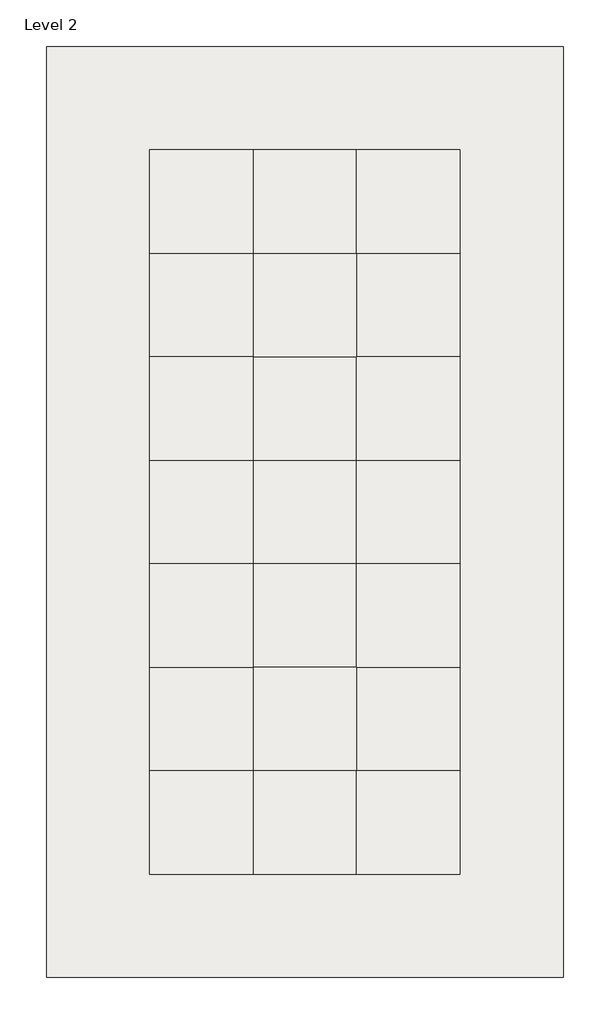
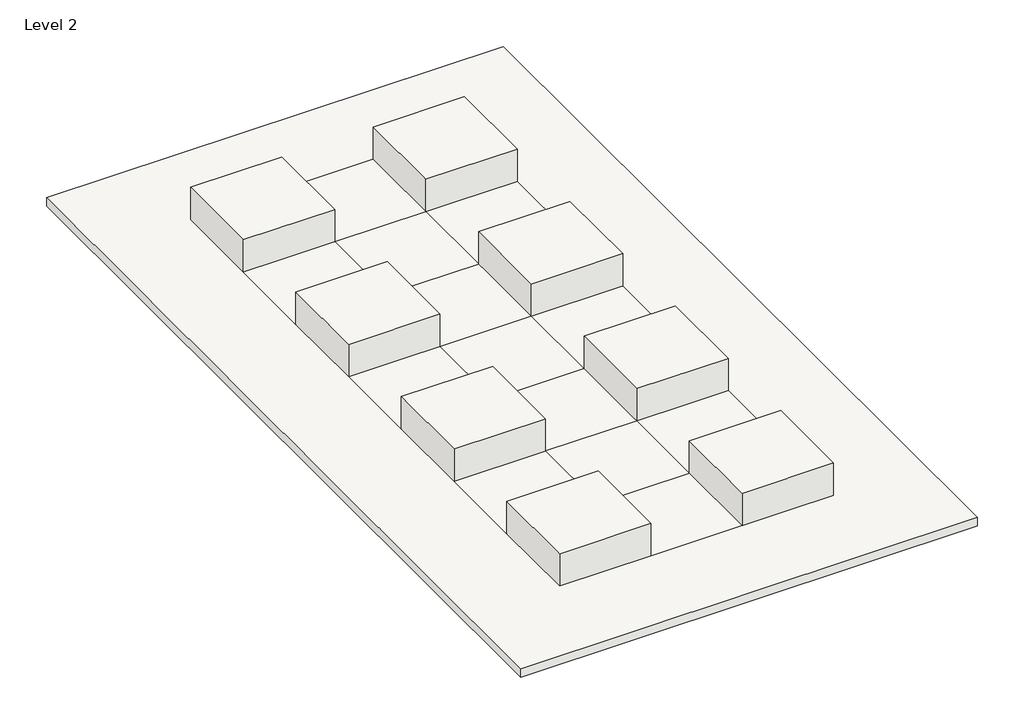
# One storey: 9 roofs.
"""IFC4 building model written with IfcOpenShell, lengths in millimetres."""

from ifc_helpers import new_model, si_unit, origin, place, context, project, spatial, faceted_brep, element, save

model = new_model("IFC4")

# Units and contexts
model_context = context("Model", 3, world=origin())
ifc_project = project(units=[si_unit("LENGTHUNIT", "METRE", prefix="MILLI")], contexts=[model_context])

# Site, building, storey
site = spatial("IfcSite", under=ifc_project)
building = spatial("IfcBuilding", under=site)
storey = spatial("IfcBuildingStorey", under=building, Name="Level 2", Elevation=8000.0)

# Roofs
placement = place(None, origin())
element("IfcRoof", 1, ObjectType="Bauder_RoofCoveringSystem_IntensiveGreenRoofSystem", at=placement, inside=storey, context=model_context, shape_type="Brep", body=[
    faceted_brep([(-674.7340554, 1676.2074539, 8000.0), (1325.2659446, 1676.2074539, 8000.0), (1325.2659446, -323.7925461, 8000.0), (-674.7340554, -323.7925461, 8000.0), (1325.2659446, 1676.2074539, 8949.8), (-674.7340554, 1676.2074539, 8949.8), (-674.7340554, -323.7925461, 8949.8), (1325.2659446, -323.7925461, 8949.8), (1325.2659446, 1676.2074539, 8200.0), (-674.7340554, 1676.2074539, 8200.0), (-674.7340554, -323.7925461, 8200.0), (1325.2659446, -323.7925461, 8200.0)], [[[0, 1, 2, 3]], [[4, 5, 6, 7]], [[5, 4, 8, 1, 0, 9]], [[6, 5, 9, 0, 3, 10]], [[7, 6, 10, 3, 2, 11]], [[4, 7, 11, 2, 1, 8]]]),
])
element("IfcRoof", 2, ObjectType="Bauder_RoofCoveringSystem_IntensiveGreenRoofSystem", at=placement, inside=storey, context=model_context, shape_type="Brep", body=[
    faceted_brep([(3325.2659446, 1676.2074539, 8000.0), (5325.2659446, 1676.2074539, 8000.0), (5325.2659446, -323.7925461, 8000.0), (3325.2659446, -323.7925461, 8000.0), (5325.2659446, 1676.2074539, 8949.8), (3325.2659446, 1676.2074539, 8949.8), (3325.2659446, -323.7925461, 8949.8), (5325.2659446, -323.7925461, 8949.8), (5325.2659446, 1676.2074539, 8200.0), (3325.2659446, 1676.2074539, 8200.0), (3325.2659446, -323.7925461, 8200.0), (5325.2659446, -323.7925461, 8200.0)], [[[0, 1, 2, 3]], [[4, 5, 6, 7]], [[5, 4, 8, 1, 0, 9]], [[6, 5, 9, 0, 3, 10]], [[7, 6, 10, 3, 2, 11]], [[4, 7, 11, 2, 1, 8]]]),
])
element("IfcRoof", 3, ObjectType="Bauder_RoofCoveringSystem_IntensiveGreenRoofSystem", at=placement, inside=storey, context=model_context, shape_type="Brep", body=[
    faceted_brep([(3325.2659446, -2323.7925461, 8000.0), (5325.2659446, -2323.7925461, 8000.0), (5325.2659446, -4323.7925461, 8000.0), (3325.2659446, -4323.7925461, 8000.0), (5325.2659446, -2323.7925461, 8949.8), (3325.2659446, -2323.7925461, 8949.8), (3325.2659446, -4323.7925461, 8949.8), (5325.2659446, -4323.7925461, 8949.8), (5325.2659446, -2323.7925461, 8200.0), (3325.2659446, -2323.7925461, 8200.0), (3325.2659446, -4323.7925461, 8200.0), (5325.2659446, -4323.7925461, 8200.0)], [[[0, 1, 2, 3]], [[4, 5, 6, 7]], [[5, 4, 8, 1, 0, 9]], [[6, 5, 9, 0, 3, 10]], [[7, 6, 10, 3, 2, 11]], [[4, 7, 11, 2, 1, 8]]]),
])
element("IfcRoof", 4, ObjectType="Bauder_RoofCoveringSystem_IntensiveGreenRoofSystem", at=placement, inside=storey, context=model_context, shape_type="Brep", body=[
    faceted_brep([(3325.2659446, -6323.7925461, 8000.0), (5325.2659446, -6323.7925461, 8000.0), (5325.2659446, -8323.7925461, 8000.0), (3325.2659446, -8323.7925461, 8000.0), (5325.2659446, -6323.7925461, 8949.8), (3325.2659446, -6323.7925461, 8949.8), (3325.2659446, -8323.7925461, 8949.8), (5325.2659446, -8323.7925461, 8949.8), (5325.2659446, -6323.7925461, 8200.0), (3325.2659446, -6323.7925461, 8200.0), (3325.2659446, -8323.7925461, 8200.0), (5325.2659446, -8323.7925461, 8200.0)], [[[0, 1, 2, 3]], [[4, 5, 6, 7]], [[5, 4, 8, 1, 0, 9]], [[6, 5, 9, 0, 3, 10]], [[7, 6, 10, 3, 2, 11]], [[4, 7, 11, 2, 1, 8]]]),
])
element("IfcRoof", 5, ObjectType="Bauder_RoofCoveringSystem_IntensiveGreenRoofSystem", at=placement, inside=storey, context=model_context, shape_type="Brep", body=[
    faceted_brep([(3325.2659446, -10323.7925461, 8000.0), (5325.2659446, -10323.7925461, 8000.0), (5325.2659446, -12323.7925461, 8000.0), (3325.2659446, -12323.7925461, 8000.0), (5325.2659446, -10323.7925461, 8949.8), (3325.2659446, -10323.7925461, 8949.8), (3325.2659446, -12323.7925461, 8949.8), (5325.2659446, -12323.7925461, 8949.8), (5325.2659446, -10323.7925461, 8200.0), (3325.2659446, -10323.7925461, 8200.0), (3325.2659446, -12323.7925461, 8200.0), (5325.2659446, -12323.7925461, 8200.0)], [[[0, 1, 2, 3]], [[4, 5, 6, 7]], [[5, 4, 8, 1, 0, 9]], [[6, 5, 9, 0, 3, 10]], [[7, 6, 10, 3, 2, 11]], [[4, 7, 11, 2, 1, 8]]]),
])
element("IfcRoof", 6, ObjectType="Bauder_RoofCoveringSystem_IntensiveGreenRoofSystem", at=placement, inside=storey, context=model_context, shape_type="Brep", body=[
    faceted_brep([(-674.7340554, -10323.7925461, 8000.0), (1325.2659446, -10323.7925461, 8000.0), (1325.2659446, -12323.7925461, 8000.0), (-674.7340554, -12323.7925461, 8000.0), (1325.2659446, -10323.7925461, 8949.8), (-674.7340554, -10323.7925461, 8949.8), (-674.7340554, -12323.7925461, 8949.8), (1325.2659446, -12323.7925461, 8949.8), (1325.2659446, -10323.7925461, 8200.0), (-674.7340554, -10323.7925461, 8200.0), (-674.7340554, -12323.7925461, 8200.0), (1325.2659446, -12323.7925461, 8200.0)], [[[0, 1, 2, 3]], [[4, 5, 6, 7]], [[5, 4, 8, 1, 0, 9]], [[6, 5, 9, 0, 3, 10]], [[7, 6, 10, 3, 2, 11]], [[4, 7, 11, 2, 1, 8]]]),
])
element("IfcRoof", 7, ObjectType="Bauder_RoofCoveringSystem_IntensiveGreenRoofSystem", at=placement, inside=storey, context=model_context, shape_type="Brep", body=[
    faceted_brep([(-674.7340554, -6323.7925461, 8000.0), (1325.2659446, -6323.7925461, 8000.0), (1325.2659446, -8323.7925461, 8000.0), (-674.7340554, -8323.7925461, 8000.0), (1325.2659446, -6323.7925461, 8949.8), (-674.7340554, -6323.7925461, 8949.8), (-674.7340554, -8323.7925461, 8949.8), (1325.2659446, -8323.7925461, 8949.8), (1325.2659446, -6323.7925461, 8200.0), (-674.7340554, -6323.7925461, 8200.0), (-674.7340554, -8323.7925461, 8200.0), (1325.2659446, -8323.7925461, 8200.0)], [[[0, 1, 2, 3]], [[4, 5, 6, 7]], [[5, 4, 8, 1, 0, 9]], [[6, 5, 9, 0, 3, 10]], [[7, 6, 10, 3, 2, 11]], [[4, 7, 11, 2, 1, 8]]]),
])
element("IfcRoof", 8, ObjectType="Bauder_RoofCoveringSystem_IntensiveGreenRoofSystem", at=placement, inside=storey, context=model_context, shape_type="Brep", body=[
    faceted_brep([(-674.7340554, -2323.7925461, 8000.0), (1325.2659446, -2323.7925461, 8000.0), (1325.2659446, -4323.7925461, 8000.0), (-674.7340554, -4323.7925461, 8000.0), (1325.2659446, -2323.7925461, 8949.8), (-674.7340554, -2323.7925461, 8949.8), (-674.7340554, -4323.7925461, 8949.8), (1325.2659446, -4323.7925461, 8949.8), (1325.2659446, -2323.7925461, 8200.0), (-674.7340554, -2323.7925461, 8200.0), (-674.7340554, -4323.7925461, 8200.0), (1325.2659446, -4323.7925461, 8200.0)], [[[0, 1, 2, 3]], [[4, 5, 6, 7]], [[5, 4, 8, 1, 0, 9]], [[6, 5, 9, 0, 3, 10]], [[7, 6, 10, 3, 2, 11]], [[4, 7, 11, 2, 1, 8]]]),
])
element("IfcRoof", 9, ObjectType="Roof_Concrete-200mm", at=placement, inside=storey, context=model_context, shape_type="Brep", body=[
    faceted_brep([(-2674.7340554, -14323.7925461, 8200.0), (-2674.7340554, -14323.7925461, 8000.0), (7325.2659446, -14323.7925461, 8000.0), (7325.2659446, -14323.7925461, 8200.0), (-2674.7340554, 3676.2074539, 8200.0), (-2674.7340554, 3676.2074539, 8000.0), (7325.2659446, 3676.2074539, 8200.0), (7325.2659446, 3676.2074539, 8000.0), (3325.2659446, 1676.2074539, 8200.0), (1325.2659446, 1676.2074539, 8200.0), (1325.2659446, -323.7925461, 8200.0), (3325.2659446, -323.7925461, 8200.0), (1325.2659446, 1676.2074539, 8000.0), (3325.2659446, 1676.2074539, 8000.0), (3325.2659446, -323.7925461, 8000.0), (1325.2659446, -323.7925461, 8000.0), (1325.2659446, -2323.7925461, 8200.0), (-674.7340554, -323.7925461, 8200.0), (-674.7340554, -2323.7925461, 8200.0), (3325.2659446, -2323.7925461, 8200.0), (5325.2659446, -2323.7925461, 8200.0), (5325.2659446, -323.7925461, 8200.0), (-674.7340554, -2323.7925461, 8000.0), (-674.7340554, -323.7925461, 8000.0), (1325.2659446, -2323.7925461, 8000.0), (3325.2659446, -2323.7925461, 8000.0), (5325.2659446, -323.7925461, 8000.0), (5325.2659446, -2323.7925461, 8000.0), (1325.2659446, -4323.7925461, 8200.0), (3325.2659446, -4323.7925461, 8200.0), (3325.2659446, -4323.7925461, 8000.0), (1325.2659446, -4323.7925461, 8000.0), (1325.2659446, -6323.7925461, 8200.0), (-674.7340554, -4323.7925461, 8200.0), (-674.7340554, -6323.7925461, 8200.0), (5325.2659446, -6323.7925461, 8200.0), (5325.2659446, -4323.7925461, 8200.0), (3325.2659446, -6323.7925461, 8200.0), (-674.7340554, -6323.7925461, 8000.0), (-674.7340554, -4323.7925461, 8000.0), (1325.2659446, -6323.7925461, 8000.0), (3325.2659446, -6323.7925461, 8000.0), (5325.2659446, -4323.7925461, 8000.0), (5325.2659446, -6323.7925461, 8000.0), (1325.2659446, -12323.7925461, 8200.0), (3325.2659446, -12323.7925461, 8200.0), (3325.2659446, -10323.7925461, 8200.0), (1325.2659446, -10323.7925461, 8200.0), (3325.2659446, -12323.7925461, 8000.0), (1325.2659446, -12323.7925461, 8000.0), (1325.2659446, -10323.7925461, 8000.0), (3325.2659446, -10323.7925461, 8000.0), (1325.2659446, -8323.7925461, 8200.0), (-674.7340554, -8323.7925461, 8200.0), (-674.7340554, -10323.7925461, 8200.0), (3325.2659446, -8323.7925461, 8200.0), (5325.2659446, -10323.7925461, 8200.0), (5325.2659446, -8323.7925461, 8200.0), (-674.7340554, -10323.7925461, 8000.0), (-674.7340554, -8323.7925461, 8000.0), (1325.2659446, -8323.7925461, 8000.0), (3325.2659446, -8323.7925461, 8000.0), (5325.2659446, -8323.7925461, 8000.0), (5325.2659446, -10323.7925461, 8000.0), (-674.7340554, 1676.2074539, 8000.0), (-674.7340554, 1676.2074539, 8200.0), (5325.2659446, 1676.2074539, 8200.0), (5325.2659446, 1676.2074539, 8000.0), (5325.2659446, -12323.7925461, 8000.0), (5325.2659446, -12323.7925461, 8200.0), (-674.7340554, -12323.7925461, 8000.0), (-674.7340554, -12323.7925461, 8200.0)], [[[0, 1, 2, 3]], [[1, 0, 4, 5]], [[6, 7, 5, 4]], [[3, 2, 7, 6]], [[8, 9, 10, 11]], [[12, 13, 14, 15]], [[16, 10, 17, 18]], [[11, 10, 16, 19]], [[20, 21, 11, 19]], [[22, 23, 15, 24]], [[15, 14, 25, 24]], [[25, 14, 26, 27]], [[19, 16, 28, 29]], [[24, 25, 30, 31]], [[32, 28, 33, 34]], [[35, 36, 29, 37]], [[38, 39, 31, 40]], [[41, 30, 42, 43]], [[44, 45, 46, 47]], [[48, 49, 50, 51]], [[47, 52, 53, 54]], [[47, 46, 55, 52]], [[56, 57, 55, 46]], [[58, 59, 60, 50]], [[51, 50, 60, 61]], [[51, 61, 62, 63]], [[52, 55, 37, 32]], [[29, 28, 32, 37]], [[61, 60, 40, 41]], [[31, 30, 41, 40]], [[9, 12, 15, 10]], [[10, 15, 23, 17]], [[17, 23, 64, 65]], [[12, 9, 65, 64]], [[66, 67, 26, 21]], [[21, 26, 14, 11]], [[11, 14, 13, 8]], [[67, 66, 8, 13]], [[20, 27, 42, 36]], [[36, 42, 30, 29]], [[29, 30, 25, 19]], [[27, 20, 19, 25]], [[16, 24, 31, 28]], [[28, 31, 39, 33]], [[33, 39, 22, 18]], [[24, 16, 18, 22]], [[32, 40, 60, 52]], [[52, 60, 59, 53]], [[53, 59, 38, 34]], [[40, 32, 34, 38]], [[35, 43, 62, 57]], [[57, 62, 61, 55]], [[55, 61, 41, 37]], [[43, 35, 37, 41]], [[56, 63, 68, 69]], [[69, 68, 48, 45]], [[45, 48, 51, 46]], [[63, 56, 46, 51]], [[47, 50, 49, 44]], [[44, 49, 70, 71]], [[71, 70, 58, 54]], [[50, 47, 54, 58]], [[4, 0, 3, 6], [9, 8, 66, 21, 20, 36, 35, 57, 56, 69, 45, 44, 71, 54, 53, 34, 33, 18, 17, 65]], [[7, 2, 1, 5], [13, 12, 64, 23, 22, 39, 38, 59, 58, 70, 49, 48, 68, 63, 62, 43, 42, 27, 26, 67]]]),
])

save(model, "model.ifc")

# Revit data of these elements
# Type "Bauder_RoofCoveringSystem_IntensiveGreenRoofSystem"
#   Keynote = "Q37"
#   Type IFC Predefined Type = "FLAT_ROOF"
#   Export Type to IFC As = "IfcRoofType"
#   Model = "Bauder Intensive Landscaping and Substrate - Intensive Green Roof System"
#   Manufacturer = "Bauder Ltd"
#   Type Comments = "Intensive Green Roof System"
#   URL = "http://www.bauder.co.uk/"
#   Description = "Bauder Intensive GreenRoof system incorporating Intensive Landscaping with Intensive Substrate, Filter Fleece, Mineral Drain, DSE60 Polyethylene Drainage and Protection Layer, FSM 1100 protection mat and PE Foil Polyethylene Separation-Slip Layer"
#   Assembly Code = "B3010"
#   NBSDescription = "Intensive green roof system"
#   NBSReference = "45-40-47/110"
#   BIMObjectName = "Bauder_RoofCoveringSystem_IntensiveGreenRoofSystem"
#   AccessibilityPerformance = "n/a"
#   CodePerformance = "n/a"
#   Color = "n/a"
#   Constituents = "n/a"
#   DurationUnit = "Year"
#   ExpectedLife = "n/a"
#   Features = "This BIM Object must be supported by a project specific specification from Bauder, incorporating system build-up, detail design and performance calculations if a full Bauder system guarantee is required. Please contact your local Bauder Representative or technical@bauder.co.uk"
#   Finish = "n/a"
#   Grade = "n/a"
#   Material = "n/a"
#   ModelReference = "Bauder Intensive Landscaping and Substrate - Intensive Green Roof System"
#   Name = "RoofCoveringSystem_Bauder_IntensiveGreenRoofSystem"
#   ReplacementCost = "n/a"
#   Shape = "n/a"
#   Size = "n/a"
#   SustainabilityPerformance = "Bauder Germany ISO14001: Certificate No.: 70499/03-15 e, Bauder UK ISO14001:Certificate No. 19ACM6595R, EN1271, BREEAM Credits Available"
#   WarrantyDescription = "Guarantee options could include ‘Product’, ‘Product and Workmanship’ and ‘Product, Workmanship and Design’ Guarantees. All guarantees available for this system are subject to the works being carried out in accordance with the Bauder specification and being installed by a Bauder Approved installer. For full details and further information regarding guarantees and alternative systems please contact your local Bauder Representative or technical@bauder.co.uk"
#   WarrantyDurationLabor = "n/a"
#   WarrantyDurationParts = "n/a\r\nn/a"
#   WarrantyDurationUnit = "Year"
#   WarrantyGuarantorLabor = "n/a"
#   WarrantyGuarantorParts = "technical@bauder.co.uk"
#   Certification = "n/a"
#   EdgeRestraints = "Perforated edge trim where required, refer to Bauder Project Specific Specification"
#   MoistureControlDrainageAncillaries = "n/a"
#   MoistureControlDrainageLayer = "Bauder DSE60 60 mm Polyethylene Drainage and Protection Layer with Bauder Mineral Drain Single size stone aggregate infill"
#   MoistureControlFilterMembrane = "Bauder Filter Fleece 1 mm Polypropylene Filter Fleece"
#   MoistureControlMoistureRetentionMat = "n/a"
#   PlantingSystemsAntierosionMat = "Jute Net where exposed, refer to Bauder Project Specific Specification"
#   PlantingSystemsPlantingMedium = "Bauder Intensive Substrate Recycled crushed brick, expanded clay shale and composted pine bark"
#   PlantingSystemsVegetation = "Bauder Intensive Landscaping"
#   PlantingSystemsVegetationBarrier = "20-40 mm Rounded-Washed Stones, refer to Bauder Project Specific Specification"
#   ProjectSpecificationAndDesign = "This BIM Object must be supported by a project specific specification from Bauder, incorporating system build-up, detail design and performance calculations if a full Bauder system warranty is required. Please contact your local Bauder Representative or technical@bauder.co.uk"
#   ProtectionProtectionLayer = "BauderGREEN FSM 1100 Protection Mat"
#   ProtectionRootBarrier = "As per project specific Bauder Specification"
#   ProtectionSeparationLayer = "2 layers of Bauder PE Foil 0.2 mm Polyethylene Separation-Slip Layer"
#   SystemManufacturer = "Bauder Ltd"
#   WarrantyConsiderations = "All guarantees available for this system are subject to the works being carried out in accordance with the Bauder specification and being installed by a Bauder Approved installer. For full details and further information regarding guarantees and alternative systems please contact your local Bauder Representative or technical@bauder.co.uk"
#   Update = "1900-12-31T23:59:59"
#   Documentation = "https://www.bauder.co.uk/technical-centre/technical-literature/system-brochures"
#   DocumentReference = "http://www.bauder.co.uk/"
#   IfcExportAs = "IfcRoofType"
#   IfcExportType = "FLAT_ROOF"
#   MethodOfMesurement = "n/a"
#   Process = "Replacement at service life intervals"
#   FireRating = "n/a"
#   _Author = "AM"
#   _AuthorizedBy = "bimstore"
#   _CreatedBy = "technical@bauder.co.uk"
#   _DistributedBy = "www.bimstore.co"
#   AssetType = "Fixed"
#   ClassificationName = "Uniclass2015"
#   ClassificationValue = "Ss_45_40_47_40"
#   CreatedBy = "technical@bauder.co.uk"
#   CreatedOn = "2023-02-10 T00:00:00"
#   DocumentationCertificates = "n/a"
#   DocumentationInstallationGuide = "https://www.bauder.co.uk/technical-centre"
#   DocumentationLiterature = "https://www.bauder.co.uk/technical-centre"
#   DocumentationMaintenance = "https://www.bauder.co.uk/technical-centre/maintenance-advice"
#   DocumentationTechnical = "https://www.bauder.co.uk/green-roofs/intensive-green-roofs"
#   ManufacturerName = "Bauder Ltd"
#   ModelNumber = "0910_INT-InS-FF-D6-F11-PE"
#   ProductionYear = "2023"
#   ReferencedStandard = "n/a"
#   SpareParts = "n/a"
#   TypeName = "Intensive Green Roof System"
#   NBSNote = "n/a"
#   NBSObjectName = "Bauder - Intensive green roof system"
#   NBSOfficeMasterTag = "n/a"
#   Ballast = "n/a"
#   CarrierMembraneFixing = "n/a"
#   CarrierMembraneType = "n/a"
#   FillToPerimeterUpstands = "n/a"
#   FilterLayer = "n/a"
#   InsulationFixing = "n/a"
#   InsulationType = "n/a"
#   LiquidAppliedWaterproofCoatingReinforcement = "n/a"
#   LiquidAppliedWaterproofCoatingSurfaceTreatment = "n/a"
#   LiquidAppliedWaterproofCoatingType = "n/a"
#   PreparationExistingSubstrates = "n/a"
#   PreparationHorizontalWork = "n/a"
#   PreparationSkirtingsAndVerticalWork = "n/a"
#   ProtectionLayer = "n/a"
#   SystemAccessories = "n/a"
#   WaterproofCoveringFirstLayerAttachment = "n/a"
#   WaterproofCoveringFirstLayerType = "n/a"
#   WaterproofCoveringIntermediateLayerAttachment = "n/a"
#   WaterproofCoveringIntermediateLayerType = "n/a"
#   WaterproofCoveringTopLayerAttachment = "n/a"
#   InsulationAttachment = "n/a"
#   IsolatingLayer = "n/a"
#   CarrierMembraneAttachment = "n/a"
#   LiquidAppliedWaterproofCoatingWearingCourse = "n/a"
#   VapourControlLayer = "n/a"
#   VapourControlLayerAttachment_Bauder = "n/a"
#   WaterproofCoveringJoints = "n/a"
#   WaterproofCoveringType = "n/a"
#   SeparatingLayer = "n/a"
#   WaterproofCoveringAccessories = "Yes"
#   WaterproofCoveringAttachment = "n/a"
#   UpperProtectionLayer = "n/a"
#   LowerProtectionLayer = "n/a"
#   WaterproofCoveringTopLayerType = "n/a"
#   DetailWorkAncillaryItems = "Detail as per project specific Bauder Specification"
#   DetailWorkCoverStrips = "Detail as per project specific Bauder Specification"
#   DetailWorkFlashings = "Detail as per project specific Bauder Specification"
#   DetailWorkSkirtingsAndUpstands = "Detail as per project specific Bauder Specification"
#   DetailWorkWeltedDrips = "Detail as per project specific Bauder Specification"
#   OverlayFixing = "n/a"
#   OverlayType = "n/a"
#   SurfaceProtection = "n/a"
#   VapourControlLayerAttachment = "n/a"
#   VapourControlLayerType = "n/a"
#   Cost = 0
#   NominalHeight = 0 mm
#   NominalLength = 0 mm
#   TotalArea = 0 m²
#   NominalDepth = 0 mm
#   IsExternal = yes
#   _BimSpecGuid = 0
#   _BSBibleVersion = 16
#   _CurrentRevision = 4
#   Layers, outside or top first: 300 mm "Bauder_Landscaping_Intensive" (function 5); 400 mm "Bauder_IntensiveSubstrate_BauderGREEN-SUB-IM-UK" (function 2); 1 mm "Bauder_FilterFleece_BauderGREEN-FV-125-100" (function 2); 40 mm "Bauder_DrainageBoard_BauderGREEN-DSE-40" (function 3); 8 mm "Bauder_ProtectionMat_BauderGREEN-FSM1100" (function 3); 200 mm "Concrete" (function 1); 0.8 mm "Bauder_SeparationAndSlipLayer_BauderGREEN-PE-02" (function 3)
# Type "Roof_Concrete-200mm"
#   Layers, outside or top first: 200 mm "Concrete" (function 1)
# Elements 1, 2, 3, 4, 5, 6, 7, 8 (IfcRoof, "Bauder_RoofCoveringSystem_IntensiveGreenRoofSystem")
#   built-in parameter 1001705 = 29.3629 (stored number, unit not read)
#   built-in parameter 1001710 = 33615
#   Phase Created = New Construction
#   Materials on its faces: "Bauder_SeparationAndSlipLayer_BauderGREEN-PE-02", "Bauder_Landscaping_Intensive"
# Element 9 (IfcRoof, "Roof_Concrete-200mm")
#   built-in parameter 1001710 = 33615
#   Phase Created = New Construction
#   Materials on its faces: "Concrete"
# Materials
#   "Bauder_Landscaping_Intensive": class "Unassigned", colour RGB 62 68 37, transparency 0, Mtrl_Author = "AM", Mtrl_AuthorizedBy = "bimstore", Mtrl_DistributedBy = "www.bimstore.co", Mtrl_AccessibilityPerformance = "n/a", Mtrl_AssetIdentifier = "Please record on commissioning", Mtrl_AssetType = "Fixed", Mtrl_BarCode = "Please record on commissioning", Mtrl_ClassificationName = "Uniclass2015", Mtrl_ClassificationValue = "n/a", Mtrl_CodePerformance = "n/a", Mtrl_Color = "n/a", Mtrl_Constituents = "n/a", Mtrl_CreatedBy = "technical@bauder.co.uk", Mtrl_CreatedOn = "2023-02-10 T00:00:00", Mtrl_DocumentationCertificates = "https://www.bimstore.co/products/intensive-green-roof-system/document/product-certificates", Mtrl_DocumentationInstallationGuide = "https://www.bimstore.co/products/intensive-green-roof-system/document/installation-guide", Mtrl_DocumentationLiterature = "https://www.bimstore.co/products/intensive-green-roof-system/document/product-literature", Mtrl_DocumentationMaintenance = "https://www.bimstore.co/products/intensive-green-roof-system/document/maintenance-information", Mtrl_DocumentationTechnical = "https://www.bimstore.co/products/intensive-green-roof-system/document/technical-data-sheet", Mtrl_DurationUnit = "Year", Mtrl_Features = "n/a", Mtrl_Finish = "n/a", Mtrl_Grade = "n/a", Mtrl_InstallationDate = "Please record on commissioning", Mtrl_ManufacturerName = "Bauder Ltd", Mtrl_Material = "n/a", Mtrl_ModelNumber = "Intensive", Mtrl_ModelReference = "Landscaping", Mtrl_ProductionYear = "2023", Mtrl_ReferencedStandard = "n/a", Mtrl_Shape = "n/a", Mtrl_Size = "n/a", Mtrl_SpareParts = "n/a", Mtrl_TypeName = "Intensive", Mtrl_WarrantyDescription = "n/a", Mtrl_WarrantyDurationUnit = "Year", Mtrl_WarrantyGuarantorLabor = "n/a", Mtrl_WarrantyGuarantorParts = "technical@bauder.co.uk", Mtrl_WarrantyStartDate = "Please record on commissioning", Mtrl_IfcExportAs = "IfcRoofType", Mtrl_IfcExportType = "FLAT_ROOF", Mtrl_BIMObjectName = "Bauder_Landscaping_Intensive", Mtrl_NBSDescription = "n/a", Mtrl_NBSNote = "n/a", Mtrl_NBSObjectName = "n/a", Mtrl_NBSOfficeMasterTag = "n/a", Mtrl_NBSReference = "Q37", Mtrl_Ballast = "n/a", Mtrl_CarrierMembraneAttachment = "n/a", Mtrl_CarrierMembraneFixing = "n/a", Mtrl_CarrierMembraneType = "n/a", Mtrl_Certification = "Comply with GRO Green Roof Code of Practice and FLL Standards", Mtrl_DetailWorkAncillaryItems = "Detail as per project specific Bauder Specification", Mtrl_DetailWorkCoverStrips = "Detail as per project specific Bauder Specification", Mtrl_DetailWorkFlashings = "Detail as per project specific Bauder Specification", Mtrl_DetailWorkSkirtingsAndUpstands = "Detail as per project specific Bauder Specification", Mtrl_DetailWorkWeltedDrips = "Detail as per project specific Bauder Specification", Mtrl_EdgeRestraints = "Detail as per project specific Bauder Specification", Mtrl_FillToPerimeterUpstands = "n/a", Mtrl_FilterLayer = "n/a", Mtrl_InsulationAttachment = "As per project specific Bauder Specification", Mtrl_InsulationFixing = "As per project specific Bauder Specification", Mtrl_InsulationType = "As per project specific Bauder Specification", Mtrl_IsolatingLayer = "n/a", Mtrl_LiquidAppliedWaterproofCoatingReinforcement = "n/a", Mtrl_LiquidAppliedWaterproofCoatingSurfaceTreatment = "As per project specific Bauder Specification", Mtrl_LiquidAppliedWaterproofCoatingType = "As per project specific Bauder Specification", Mtrl_LiquidAppliedWaterproofCoatingWearingCourse = "As per project specific Bauder Specification", Mtrl_LowerProtectionLayer = "n/a", Mtrl_MoistureControlDrainageAncillaries = "n/a", Mtrl_MoistureControlDrainageLayer = "n/a", Mtrl_MoistureControlFilterMembrane = "n/a", Mtrl_MoistureControlMoistureRetentionMat = "n/a", Mtrl_OverlayFixing = "n/a", Mtrl_OverlayType = "n/a", Mtrl_PlantingSystemsAntierosionMat = "n/a", Mtrl_PlantingSystemsPlantingMedium = "As per project specific Bauder Specification", Mtrl_PlantingSystemsVegetation = "As per project specific Bauder Specification", Mtrl_PlantingSystemsVegetationBarrier = "As per project specific Bauder Specification", Mtrl_PreparationExistingSubstrates = "n/a", Mtrl_PreparationHorizontalWork = "n/a", Mtrl_PreparationSkirtingsAndVerticalWork = "n/a", Mtrl_ProjectSpecificationAndDesign = "This BIM Object must be supported by a project specific specification from Bauder, incorporating system build-up, detail design and performance calculations if a full Bauder system warranty is required. Please contact your local Bauder Representative or technical@bauder.co.uk", Mtrl_ProtectionLayer = "n/a", Mtrl_ProtectionProtectionLayer = "n/a", Mtrl_ProtectionRootBarrier = "As per project specific Bauder Specification", Mtrl_ProtectionSeparationLayer = "n/a", Mtrl_SeparatingLayer = "n/a", Mtrl_SurfaceProtection = "n/a", Mtrl_SystemAccessories = "n/a", Mtrl_SystemManufacturer = "Bauder Ltd", Mtrl_Update = "1900-12-31 T23:59:59", Mtrl_UpperProtectionLayer = "n/a", Mtrl_VapourControlLayerAttachment = "As per project specific Bauder Specification", Mtrl_VapourControlLayerAttachment_Bauder = "As per project specific Bauder Specification", Mtrl_VapourControlLayerType = "As per project specific Bauder Specification", Mtrl_WarrantyConsiderations = "All guarantees available for this system are subject to the works being carried out in accordance with the Bauder specification and being installed by a Bauder Approved installer. For full details and further information regarding guarantees and alternative systems please contact your local Bauder Representative or technical@bauder.co.uk", Mtrl_WaterproofCoveringAccessories = "As per project specific Bauder Specification", Mtrl_WaterproofCoveringAttachment = "As per project specific Bauder Specification", Mtrl_WaterproofCoveringFirstLayerAttachment = "As per project specific Bauder Specification", Mtrl_WaterproofCoveringFirstLayerType = "As per project specific Bauder Specification", Mtrl_WaterproofCoveringIntermediateLayerAttachment = "As per project specific Bauder Specification", Mtrl_WaterproofCoveringIntermediateLayerType = "As per project specific Bauder Specification", Mtrl_WaterproofCoveringJoints = "As per project specific Bauder Specification", Mtrl_WaterproofCoveringTopLayerAttachment = "As per project specific Bauder Specification", Mtrl_WaterproofCoveringTopLayerType = "As per project specific Bauder Specification", Mtrl_WaterproofCoveringType = "As per project specific Bauder Specification", Cost = 0, Mtrl_ReplacementCost = 0, Mtrl_NominalDepth = 0 mm, Mtrl_NominalHeight = 0 mm, Mtrl_NominalLength = 0 mm, Mtrl_BimSpecGuid = 0, Mtrl_BSBibleVersion = 17, Mtrl_CurrentRevision = 2, Mtrl_ExpectedLife = 0, Mtrl_SerialNumber = 0, Mtrl_WarrantyDurationLabor = 0, Mtrl_WarrantyDurationParts = 0
#   "Bauder_IntensiveSubstrate_BauderGREEN-SUB-IM-UK": class "Unassigned", colour RGB 255 255 255, transparency 0, Mtrl_Author = "AM", Mtrl_AuthorizedBy = "bimstore", Mtrl_DistributedBy = "www.bimstore.co", Mtrl_AccessibilityPerformance = "n/a", Mtrl_AssetIdentifier = "Please record on commissioning", Mtrl_AssetType = "Fixed", Mtrl_BarCode = "Please record on commissioning", Mtrl_ClassificationName = "Uniclass2015", Mtrl_ClassificationValue = "n/a", Mtrl_CodePerformance = "n/a", Mtrl_Color = "n/a", Mtrl_Constituents = "n/a", Mtrl_CreatedBy = "technical@bauder.co.uk", Mtrl_CreatedOn = "2023-02-10 T00:00:00", Mtrl_DocumentationCertificates = "https://www.bimstore.co/products/intensive-green-roof-system/document/product-certificates", Mtrl_DocumentationInstallationGuide = "https://www.bimstore.co/products/intensive-green-roof-system/document/installation-guide", Mtrl_DocumentationLiterature = "https://www.bimstore.co/products/intensive-green-roof-system/document/product-literature", Mtrl_DocumentationMaintenance = "https://www.bimstore.co/products/intensive-green-roof-system/document/maintenance-information", Mtrl_DocumentationTechnical = "https://www.bimstore.co/products/intensive-green-roof-system/document/technical-data-sheet", Mtrl_DurationUnit = "Year", Mtrl_Features = "n/a", Mtrl_Finish = "n/a", Mtrl_Grade = "n/a", Mtrl_InstallationDate = "Please record on commissioning", Mtrl_ManufacturerName = "Bauder Ltd", Mtrl_Material = "Expanded Clay Aggregate", Mtrl_ModelNumber = "BauderGREEN-SUB-IM-UK", Mtrl_ModelReference = "Intensive Substrate", Mtrl_ProductionYear = "2023", Mtrl_ReferencedStandard = "n/a", Mtrl_Shape = "n/a", Mtrl_Size = "n/a", Mtrl_SpareParts = "n/a", Mtrl_TypeName = "BauderGREEN-SUB-IM-UK", Mtrl_WarrantyDescription = "As part of Bauder system guarantee, per specification", Mtrl_WarrantyDurationUnit = "Year", Mtrl_WarrantyGuarantorLabor = "n/a", Mtrl_WarrantyGuarantorParts = "technical@bauder.co.uk", Mtrl_WarrantyStartDate = "Please record on commissioning", Mtrl_IfcExportAs = "IfcRoofType", Mtrl_IfcExportType = "FLAT_ROOF", Mtrl_BIMObjectName = "Bauder_IntensiveSubstrate_BauderGREEN-SUB-IM-UK", Mtrl_NBSDescription = "n/a", Mtrl_NBSNote = "n/a", Mtrl_NBSObjectName = "n/a", Mtrl_NBSOfficeMasterTag = "n/a", Mtrl_NBSReference = "Q37", Mtrl_Ballast = "n/a", Mtrl_CarrierMembraneAttachment = "n/a", Mtrl_CarrierMembraneFixing = "n/a", Mtrl_CarrierMembraneType = "n/a", Mtrl_Certification = "Comply with GRO Green Roof Code of Practice and FLL Standards", Mtrl_DetailWorkAncillaryItems = "Detail as per project specific Bauder Specification", Mtrl_DetailWorkCoverStrips = "Detail as per project specific Bauder Specification", Mtrl_DetailWorkFlashings = "Detail as per project specific Bauder Specification", Mtrl_DetailWorkSkirtingsAndUpstands = "Detail as per project specific Bauder Specification", Mtrl_DetailWorkWeltedDrips = "Detail as per project specific Bauder Specification", Mtrl_EdgeRestraints = "Detail as per project specific Bauder Specification", Mtrl_FillToPerimeterUpstands = "n/a", Mtrl_FilterLayer = "n/a", Mtrl_InsulationAttachment = "As per project specific Bauder Specification", Mtrl_InsulationFixing = "As per project specific Bauder Specification", Mtrl_InsulationType = "As per project specific Bauder Specification", Mtrl_IsolatingLayer = "n/a", Mtrl_LiquidAppliedWaterproofCoatingReinforcement = "As per project specific Bauder Specification", Mtrl_LiquidAppliedWaterproofCoatingSurfaceTreatment = "As per project specific Bauder Specification", Mtrl_LiquidAppliedWaterproofCoatingType = "As per project specific Bauder Specification", Mtrl_LiquidAppliedWaterproofCoatingWearingCourse = "As per project specific Bauder Specification", Mtrl_LowerProtectionLayer = "n/a", Mtrl_MoistureControlDrainageAncillaries = "n/a", Mtrl_MoistureControlDrainageLayer = "n/a", Mtrl_MoistureControlFilterMembrane = "n/a", Mtrl_MoistureControlMoistureRetentionMat = "n/a", Mtrl_OverlayFixing = "n/a", Mtrl_OverlayType = "n/a", Mtrl_PlantingSystemsAntierosionMat = "n/a", Mtrl_PlantingSystemsPlantingMedium = "As per project specific Bauder Specification", Mtrl_PlantingSystemsVegetation = "As per project specific Bauder Specification", Mtrl_PlantingSystemsVegetationBarrier = "As per project specific Bauder Specification", Mtrl_PreparationExistingSubstrates = "n/a", Mtrl_PreparationHorizontalWork = "n/a", Mtrl_PreparationSkirtingsAndVerticalWork = "n/a", Mtrl_ProjectSpecificationAndDesign = "This BIM Object must be supported by a project specific specification from Bauder, incorporating system build-up, detail design and performance calculations if a full Bauder system warranty is required. Please contact your local Bauder Representative or technical@bauder.co.uk", Mtrl_ProtectionLayer = "n/a", Mtrl_ProtectionProtectionLayer = "n/a", Mtrl_ProtectionRootBarrier = "As per project specific Bauder Specification", Mtrl_ProtectionSeparationLayer = "n/a", Mtrl_SeparatingLayer = "n/a", Mtrl_SurfaceProtection = "n/a", Mtrl_SystemAccessories = "n/a", Mtrl_SystemManufacturer = "Bauder Ltd", Mtrl_Update = "1900-12-31 T23:59:59", Mtrl_UpperProtectionLayer = "n/a", Mtrl_VapourControlLayerAttachment = "As per project specific Bauder Specification", Mtrl_VapourControlLayerAttachment_Bauder = "As per project specific Bauder Specification", Mtrl_VapourControlLayerType = "As per project specific Bauder Specification", Mtrl_WarrantyConsiderations = "All guarantees available for this system are subject to the works being carried out in accordance with the Bauder specification and being installed by a Bauder Approved installer. For full details and further information regarding guarantees and alternative systems please contact your local Bauder Representative or technical@bauder.co.uk", Mtrl_WaterproofCoveringAccessories = "As per project specific Bauder Specification", Mtrl_WaterproofCoveringAttachment = "As per project specific Bauder Specification", Mtrl_WaterproofCoveringFirstLayerAttachment = "As per project specific Bauder Specification", Mtrl_WaterproofCoveringFirstLayerType = "As per project specific Bauder Specification", Mtrl_WaterproofCoveringIntermediateLayerAttachment = "As per project specific Bauder Specification", Mtrl_WaterproofCoveringIntermediateLayerType = "As per project specific Bauder Specification", Mtrl_WaterproofCoveringJoints = "As per project specific Bauder Specification", Mtrl_WaterproofCoveringTopLayerAttachment = "As per project specific Bauder Specification", Mtrl_WaterproofCoveringTopLayerType = "As per project specific Bauder Specification", Mtrl_WaterproofCoveringType = "As per project specific Bauder Specification", Cost = 0, Mtrl_ReplacementCost = 0, Mtrl_NominalDepth = 200 mm, Mtrl_NominalHeight = 0 mm, Mtrl_NominalLength = 0 mm, Mtrl_BimSpecGuid = 0, Mtrl_BSBibleVersion = 17, Mtrl_CurrentRevision = 2, Mtrl_ExpectedLife = 0, Mtrl_SerialNumber = 0, Mtrl_WarrantyDurationLabor = 0, Mtrl_WarrantyDurationParts = 0
#   "Bauder_FilterFleece_BauderGREEN-FV-125-100": class "Unassigned", colour RGB 255 255 255, transparency 0, Mtrl_Author = "AM", Mtrl_AuthorizedBy = "bimstore", Mtrl_DistributedBy = "www.bimstore.co", Mtrl_AccessibilityPerformance = "n/a", Mtrl_AssetIdentifier = "Please record on commissioning", Mtrl_AssetType = "Fixed", Mtrl_BarCode = "Please record on commissioning", Mtrl_ClassificationName = "Uniclass2015", Mtrl_ClassificationValue = "n/a", Mtrl_CodePerformance = "n/a", Mtrl_Color = "n/a", Mtrl_Constituents = "n/a", Mtrl_CreatedBy = "technical@bauder.co.uk", Mtrl_CreatedOn = "2023-02-10 T00:00:00", Mtrl_DocumentationCertificates = "https://www.bimstore.co/products/extensive-green-roof-system-wildflower-blanket/document/product-certificates", Mtrl_DocumentationInstallationGuide = "https://www.bimstore.co/products/extensive-green-roof-system-wildflower-blanket/document/installation-guide", Mtrl_DocumentationLiterature = "https://www.bimstore.co/products/intensive-green-roof-system/document/product-literature", Mtrl_DocumentationMaintenance = "https://www.bimstore.co/products/extensive-green-roof-system-wildflower-blanket/document/maintenance-information", Mtrl_DocumentationTechnical = "https://www.bimstore.co/products/extensive-green-roof-system-wildflower-blanket/document/technical-data-sheet", Mtrl_DurationUnit = "Year", Mtrl_Features = "n/a", Mtrl_Finish = "n/a", Mtrl_Grade = "n/a", Mtrl_InstallationDate = "Please record on commissioning", Mtrl_ManufacturerName = "Bauder Ltd", Mtrl_Material = "Polypropylene Fleece", Mtrl_ModelNumber = "BauderGREEN-FV-125-100", Mtrl_ModelReference = "Filter Fleece", Mtrl_ProductionYear = "2023", Mtrl_ReferencedStandard = "n/a", Mtrl_Shape = "n/a", Mtrl_Size = "n/a", Mtrl_SpareParts = "n/a", Mtrl_TypeName = "BauderGREEN-FV-125-100", Mtrl_WarrantyDescription = "As part of Bauder system guarantee, per specification", Mtrl_WarrantyDurationUnit = "Year", Mtrl_WarrantyGuarantorLabor = "technical@bauder.co.uk", Mtrl_WarrantyGuarantorParts = "technical@bauder.co.uk", Mtrl_WarrantyStartDate = "Please record on commissioning", Mtrl_IfcExportAs = "IfcRoofType", Mtrl_IfcExportType = "FLAT_ROOF", Mtrl_BIMObjectName = "Bauder_FilterFleece_BauderGREEN-FV-125-100", Mtrl_NBSDescription = "n/a", Mtrl_NBSNote = "n/a", Mtrl_NBSObjectName = "n/a", Mtrl_NBSOfficeMasterTag = "n/a", Mtrl_NBSReference = "Q37", Mtrl_Ballast = "n/a", Mtrl_CarrierMembraneAttachment = "n/a", Mtrl_CarrierMembraneFixing = "n/a", Mtrl_CarrierMembraneType = "n/a", Mtrl_Certification = "Comply with GRO Green Roof Code of Practice and FLL Standards", Mtrl_DetailWorkAncillaryItems = "Detail as per project specific Bauder Specification", Mtrl_DetailWorkCoverStrips = "Detail as per project specific Bauder Specification", Mtrl_DetailWorkFlashings = "Detail as per project specific Bauder Specification", Mtrl_DetailWorkSkirtingsAndUpstands = "Detail as per project specific Bauder Specification", Mtrl_DetailWorkWeltedDrips = "Detail as per project specific Bauder Specification", Mtrl_EdgeRestraints = "Detail as per project specific Bauder Specification", Mtrl_FillToPerimeterUpstands = "n/a", Mtrl_FilterLayer = "n/a", Mtrl_InsulationAttachment = "As per project specific Bauder Specification", Mtrl_InsulationFixing = "As per project specific Bauder Specification", Mtrl_InsulationType = "As per project specific Bauder Specification", Mtrl_IsolatingLayer = "n/a", Mtrl_LiquidAppliedWaterproofCoatingReinforcement = "As per project specific Bauder Specification", Mtrl_LiquidAppliedWaterproofCoatingSurfaceTreatment = "As per project specific Bauder Specification", Mtrl_LiquidAppliedWaterproofCoatingType = "As per project specific Bauder Specification", Mtrl_LiquidAppliedWaterproofCoatingWearingCourse = "As per project specific Bauder Specification", Mtrl_LowerProtectionLayer = "n/a", Mtrl_MoistureControlDrainageAncillaries = "n/a", Mtrl_MoistureControlDrainageLayer = "n/a", Mtrl_MoistureControlFilterMembrane = "n/a", Mtrl_MoistureControlMoistureRetentionMat = "n/a", Mtrl_OverlayFixing = "n/a", Mtrl_OverlayType = "n/a", Mtrl_PlantingSystemsAntierosionMat = "n/a", Mtrl_PlantingSystemsPlantingMedium = "As per project specific Bauder Specification", Mtrl_PlantingSystemsVegetation = "As per project specific Bauder Specification", Mtrl_PlantingSystemsVegetationBarrier = "As per project specific Bauder Specification", Mtrl_PreparationExistingSubstrates = "n/a", Mtrl_PreparationHorizontalWork = "n/a", Mtrl_PreparationSkirtingsAndVerticalWork = "n/a", Mtrl_ProjectSpecificationAndDesign = "This BIM Object must be supported by a project specific specification from Bauder, incorporating system build-up, detail design and performance calculations if a full Bauder system warranty is required. Please contact your local Bauder Representative or technical@bauder.co.uk", Mtrl_ProtectionLayer = "n/a", Mtrl_ProtectionProtectionLayer = "n/a", Mtrl_ProtectionRootBarrier = "As per project specific Bauder Specification", Mtrl_ProtectionSeparationLayer = "n/a", Mtrl_SeparatingLayer = "n/a", Mtrl_SurfaceProtection = "n/a", Mtrl_SystemAccessories = "n/a", Mtrl_SystemManufacturer = "Bauder Ltd", Mtrl_Update = "1900-12-31 T23:59:59", Mtrl_UpperProtectionLayer = "n/a", Mtrl_VapourControlLayerAttachment = "As per project specific Bauder Specification", Mtrl_VapourControlLayerAttachment_Bauder = "As per project specific Bauder Specification", Mtrl_VapourControlLayerType = "As per project specific Bauder Specification", Mtrl_WarrantyConsiderations = "All guarantees available for this system are subject to the works being carried out in accordance with the Bauder specification and being installed by a Bauder Approved installer. For full details and further information regarding guarantees and alternative systems please contact your local Bauder Representative or technical@bauder.co.uk", Mtrl_WaterproofCoveringAccessories = "As per project specific Bauder Specification", Mtrl_WaterproofCoveringAttachment = "As per project specific Bauder Specification", Mtrl_WaterproofCoveringFirstLayerAttachment = "As per project specific Bauder Specification", Mtrl_WaterproofCoveringFirstLayerType = "As per project specific Bauder Specification", Mtrl_WaterproofCoveringIntermediateLayerAttachment = "As per project specific Bauder Specification", Mtrl_WaterproofCoveringIntermediateLayerType = "As per project specific Bauder Specification", Mtrl_WaterproofCoveringJoints = "As per project specific Bauder Specification", Mtrl_WaterproofCoveringTopLayerAttachment = "As per project specific Bauder Specification", Mtrl_WaterproofCoveringTopLayerType = "As per project specific Bauder Specification", Mtrl_WaterproofCoveringType = "As per project specific Bauder Specification", Cost = 0, Mtrl_ReplacementCost = 0, Mtrl_NominalDepth = 1 mm, Mtrl_NominalHeight = 0 mm, Mtrl_NominalLength = 0 mm, Mtrl_BimSpecGuid = 0, Mtrl_BSBibleVersion = 17, Mtrl_CurrentRevision = 2, Mtrl_ExpectedLife = 0, Mtrl_SerialNumber = 0, Mtrl_WarrantyDurationLabor = 0, Mtrl_WarrantyDurationParts = 0
#   "Bauder_DrainageBoard_BauderGREEN-DSE-40": class "Unassigned", colour RGB 255 255 255, transparency 0, Mtrl_Author = "AM", Mtrl_AuthorizedBy = "bimstore", Mtrl_DistributedBy = "www.bimstore.co", Mtrl_AccessibilityPerformance = "n/a", Mtrl_AssetIdentifier = "Please record on commissioning", Mtrl_AssetType = "Fixed", Mtrl_BarCode = "Please record on commissioning", Mtrl_ClassificationName = "Uniclass2015", Mtrl_ClassificationValue = "Pr_65_67_78_72", Mtrl_CodePerformance = "n/a", Mtrl_Color = "n/a", Mtrl_Constituents = "n/a", Mtrl_CreatedBy = "technical@bauder.co.uk", Mtrl_CreatedOn = "2023-02-10 T00:00:00", Mtrl_DocumentationCertificates = "https://www.bimstore.co/products/extensive-green-roof-system-wildflower-blanket/document/product-certificates", Mtrl_DocumentationInstallationGuide = "https://www.bimstore.co/products/extensive-green-roof-system-wildflower-blanket/document/installation-guide", Mtrl_DocumentationLiterature = "https://www.bimstore.co/products/extensive-green-roof-system-wildflower-blanket/document/product-literature", Mtrl_DocumentationMaintenance = "https://www.bimstore.co/products/extensive-green-roof-system-wildflower-blanket/document/maintenance-information", Mtrl_DocumentationTechnical = "https://www.bimstore.co/products/extensive-green-roof-system-wildflower-blanket/document/technical-data-sheet", Mtrl_DurationUnit = "Year", Mtrl_Features = "n/a", Mtrl_Finish = "n/a", Mtrl_Grade = "n/a", Mtrl_InstallationDate = "Please record on commissioning", Mtrl_ManufacturerName = "Bauder Ltd", Mtrl_Material = "Recycled High Density Polyethylene", Mtrl_ModelNumber = "BauderGREEN-DSE-40", Mtrl_ModelReference = "Drainage Board", Mtrl_ProductionYear = "2023", Mtrl_ReferencedStandard = "n/a", Mtrl_Shape = "n/a", Mtrl_Size = "n/a", Mtrl_SpareParts = "n/a", Mtrl_TypeName = "BauderGREEN-DSE-40", Mtrl_WarrantyDescription = "As part of Bauder system guarantee, per specification", Mtrl_WarrantyDurationUnit = "Year", Mtrl_WarrantyGuarantorLabor = "technical@bauder.co.uk", Mtrl_WarrantyGuarantorParts = "technical@bauder.co.uk", Mtrl_WarrantyStartDate = "Please record on commissioning", Mtrl_IfcExportAs = "IfcRoofType", Mtrl_IfcExportType = "FLAT_ROOF", Mtrl_BIMObjectName = "Bauder_DrainageBoard_BauderGREEN-DSE-40", Mtrl_NBSDescription = "n/a", Mtrl_NBSNote = "n/a", Mtrl_NBSObjectName = "n/a", Mtrl_NBSOfficeMasterTag = "n/a", Mtrl_NBSReference = "Q37", Mtrl_Ballast = "n/a", Mtrl_CarrierMembraneAttachment = "n/a", Mtrl_CarrierMembraneFixing = "n/a", Mtrl_CarrierMembraneType = "n/a", Mtrl_Certification = "Comply with GRO Green Roof Code of Practice and FLL Standards", Mtrl_DetailWorkAncillaryItems = "Detail as per project specific Bauder Specification", Mtrl_DetailWorkCoverStrips = "Detail as per project specific Bauder Specification", Mtrl_DetailWorkFlashings = "Detail as per project specific Bauder Specification", Mtrl_DetailWorkSkirtingsAndUpstands = "Detail as per project specific Bauder Specification", Mtrl_DetailWorkWeltedDrips = "Detail as per project specific Bauder Specification", Mtrl_EdgeRestraints = "Detail as per project specific Bauder Specification", Mtrl_FillToPerimeterUpstands = "n/a", Mtrl_FilterLayer = "n/a", Mtrl_InsulationAttachment = "As per project specific Bauder Specification", Mtrl_InsulationFixing = "As per project specific Bauder Specification", Mtrl_InsulationType = "As per project specific Bauder Specification", Mtrl_IsolatingLayer = "n/a", Mtrl_LiquidAppliedWaterproofCoatingReinforcement = "As per project specific Bauder Specification", Mtrl_LiquidAppliedWaterproofCoatingSurfaceTreatment = "As per project specific Bauder Specification", Mtrl_LiquidAppliedWaterproofCoatingType = "As per project specific Bauder Specification", Mtrl_LiquidAppliedWaterproofCoatingWearingCourse = "As per project specific Bauder Specification", Mtrl_LowerProtectionLayer = "n/a", Mtrl_MoistureControlDrainageAncillaries = "n/a", Mtrl_MoistureControlDrainageLayer = "n/a", Mtrl_MoistureControlFilterMembrane = "n/a", Mtrl_MoistureControlMoistureRetentionMat = "n/a", Mtrl_OverlayFixing = "n/a", Mtrl_OverlayType = "n/a", Mtrl_PlantingSystemsAntierosionMat = "n/a", Mtrl_PlantingSystemsPlantingMedium = "As per project specific Bauder Specification", Mtrl_PlantingSystemsVegetation = "As per project specific Bauder Specification", Mtrl_PlantingSystemsVegetationBarrier = "As per project specific Bauder Specification", Mtrl_PreparationExistingSubstrates = "n/a", Mtrl_PreparationHorizontalWork = "n/a", Mtrl_PreparationSkirtingsAndVerticalWork = "n/a", Mtrl_ProjectSpecificationAndDesign = "This BIM Object must be supported by a project specific specification from Bauder, incorporating system build-up, detail design and performance calculations if a full Bauder system warranty is required. Please contact your local Bauder Representative or technical@bauder.co.uk", Mtrl_ProtectionLayer = "n/a", Mtrl_ProtectionProtectionLayer = "n/a", Mtrl_ProtectionRootBarrier = "As per project specific Bauder Specification", Mtrl_ProtectionSeparationLayer = "n/a", Mtrl_SeparatingLayer = "n/a", Mtrl_SurfaceProtection = "n/a", Mtrl_SystemAccessories = "n/a", Mtrl_SystemManufacturer = "Bauder Ltd", Mtrl_Update = "1900-12-31 T23:59:59", Mtrl_UpperProtectionLayer = "n/a", Mtrl_VapourControlLayerAttachment = "As per project specific Bauder Specification", Mtrl_VapourControlLayerAttachment_Bauder = "As per project specific Bauder Specification", Mtrl_VapourControlLayerType = "As per project specific Bauder Specification", Mtrl_WarrantyConsiderations = "All guarantees available for this system are subject to the works being carried out in accordance with the Bauder specification and being installed by a Bauder Approved installer. For full details and further information regarding guarantees and alternative systems please contact your local Bauder Representative or technical@bauder.co.uk", Mtrl_WaterproofCoveringAccessories = "As per project specific Bauder Specification", Mtrl_WaterproofCoveringAttachment = "As per project specific Bauder Specification", Mtrl_WaterproofCoveringFirstLayerAttachment = "As per project specific Bauder Specification", Mtrl_WaterproofCoveringFirstLayerType = "As per project specific Bauder Specification", Mtrl_WaterproofCoveringIntermediateLayerAttachment = "As per project specific Bauder Specification", Mtrl_WaterproofCoveringIntermediateLayerType = "As per project specific Bauder Specification", Mtrl_WaterproofCoveringJoints = "As per project specific Bauder Specification", Mtrl_WaterproofCoveringTopLayerAttachment = "As per project specific Bauder Specification", Mtrl_WaterproofCoveringTopLayerType = "As per project specific Bauder Specification", Mtrl_WaterproofCoveringType = "As per project specific Bauder Specification", Cost = 0, Mtrl_ReplacementCost = 0, Mtrl_NominalDepth = 40 mm, Mtrl_NominalHeight = 0 mm, Mtrl_NominalLength = 0 mm, Mtrl_BimSpecGuid = 0, Mtrl_BSBibleVersion = 17, Mtrl_CurrentRevision = 2, Mtrl_ExpectedLife = 0, Mtrl_SerialNumber = 0, Mtrl_WarrantyDurationLabor = 0, Mtrl_WarrantyDurationParts = 0
#   "Bauder_ProtectionMat_BauderGREEN-FSM1100": class "Unassigned", colour RGB 255 255 255, transparency 0, Mtrl_Author = "AM", Mtrl_AuthorizedBy = "bimstore", Mtrl_DistributedBy = "www.bimstore.co", Mtrl_AccessibilityPerformance = "n/a", Mtrl_AssetIdentifier = "Please record on commissioning", Mtrl_AssetType = "Fixed", Mtrl_BarCode = "Please record on commissioning", Mtrl_ClassificationName = "Uniclass2015", Mtrl_ClassificationValue = "Pr_20_96_71_64", Mtrl_CodePerformance = "n/a", Mtrl_Color = "n/a", Mtrl_Constituents = "n/a", Mtrl_CreatedBy = "technical@bauder.co.uk", Mtrl_CreatedOn = "2023-05-02 T00:00:00", Mtrl_DocumentationCertificates = "https://www.bimstore.co/products/intensive-green-roof-system/document/product-certificates", Mtrl_DocumentationInstallationGuide = "https://www.bimstore.co/products/intensive-green-roof-system/document/installation-guide", Mtrl_DocumentationLiterature = "https://www.bimstore.co/products/intensive-green-roof-system/document/product-literature", Mtrl_DocumentationMaintenance = "https://www.bimstore.co/products/intensive-green-roof-system/document/maintenance-information", Mtrl_DocumentationTechnical = "https://www.bimstore.co/products/intensive-green-roof-system/document/technical-data-sheet", Mtrl_DurationUnit = "Year", Mtrl_Features = "n/a", Mtrl_Finish = "n/a", Mtrl_Grade = "n/a", Mtrl_InstallationDate = "Please record on commissioning", Mtrl_ManufacturerName = "Bauder Ltd", Mtrl_Material = "Polyester and Polypropylene Fibre", Mtrl_ModelNumber = "BauderGREEN FSM1100", Mtrl_ModelReference = "Protection Mat", Mtrl_ProductionYear = "2023", Mtrl_ReferencedStandard = "n/a", Mtrl_Shape = "n/a", Mtrl_Size = "n/a", Mtrl_SpareParts = "n/a", Mtrl_TypeName = "BauderGREEN FSM1100", Mtrl_WarrantyDescription = "As part of Bauder system guarantee, per specification", Mtrl_WarrantyDurationUnit = "Year", Mtrl_WarrantyGuarantorLabor = "n/a", Mtrl_WarrantyGuarantorParts = "technical@bauder.co.uk", Mtrl_WarrantyStartDate = "Please record on commissioning", Mtrl_IfcExportAs = "IfcRoofType", Mtrl_IfcExportType = "FLAT_ROOF", Mtrl_BIMObjectName = "Bauder_ProtectionMat_BauderGREEN-FSM1100", Mtrl_NBSDescription = "n/a", Mtrl_NBSNote = "n/a", Mtrl_NBSObjectName = "n/a", Mtrl_NBSOfficeMasterTag = "n/a", Mtrl_NBSReference = "Q37", Mtrl_Ballast = "n/a", Mtrl_CarrierMembraneAttachment = "n/a", Mtrl_CarrierMembraneFixing = "n/a", Mtrl_CarrierMembraneType = "n/a", Mtrl_Certification = "Comply with GRO Green Roof Code of Practice and FLL Standards", Mtrl_DetailWorkAncillaryItems = "Detail as per project specific Bauder Specification", Mtrl_DetailWorkCoverStrips = "Detail as per project specific Bauder Specification", Mtrl_DetailWorkFlashings = "Detail as per project specific Bauder Specification", Mtrl_DetailWorkSkirtingsAndUpstands = "Detail as per project specific Bauder Specification", Mtrl_DetailWorkWeltedDrips = "Detail as per project specific Bauder Specification", Mtrl_EdgeRestraints = "Detail as per project specific Bauder Specification", Mtrl_FillToPerimeterUpstands = "n/a", Mtrl_FilterLayer = "n/a", Mtrl_InsulationAttachment = "As per project specific Bauder Specification", Mtrl_InsulationFixing = "As per project specific Bauder Specification", Mtrl_InsulationType = "As per project specific Bauder Specification", Mtrl_IsolatingLayer = "n/a", Mtrl_LiquidAppliedWaterproofCoatingReinforcement = "As per project specific Bauder Specification", Mtrl_LiquidAppliedWaterproofCoatingSurfaceTreatment = "As per project specific Bauder Specification", Mtrl_LiquidAppliedWaterproofCoatingType = "As per project specific Bauder Specification", Mtrl_LiquidAppliedWaterproofCoatingWearingCourse = "As per project specific Bauder Specification", Mtrl_LowerProtectionLayer = "n/a", Mtrl_MoistureControlDrainageAncillaries = "n/a", Mtrl_MoistureControlDrainageLayer = "n/a", Mtrl_MoistureControlFilterMembrane = "n/a", Mtrl_MoistureControlMoistureRetentionMat = "n/a", Mtrl_OverlayFixing = "n/a", Mtrl_OverlayType = "n/a", Mtrl_PlantingSystemsAntierosionMat = "n/a", Mtrl_PlantingSystemsPlantingMedium = "As per project specific Bauder Specification", Mtrl_PlantingSystemsVegetation = "As per project specific Bauder Specification", Mtrl_PlantingSystemsVegetationBarrier = "As per project specific Bauder Specification", Mtrl_PreparationExistingSubstrates = "n/a", Mtrl_PreparationHorizontalWork = "n/a", Mtrl_PreparationSkirtingsAndVerticalWork = "n/a", Mtrl_ProjectSpecificationAndDesign = "This BIM Object must be supported by a project specific specification from Bauder, incorporating system build-up, detail design and performance calculations if a full Bauder system warranty is required. Please contact your local Bauder Representative or technical@bauder.co.uk", Mtrl_ProtectionLayer = "n/a", Mtrl_ProtectionProtectionLayer = "n/a", Mtrl_ProtectionRootBarrier = "As per project specific Bauder Specification", Mtrl_ProtectionSeparationLayer = "n/a", Mtrl_SeparatingLayer = "n/a", Mtrl_SurfaceProtection = "n/a", Mtrl_SystemAccessories = "n/a", Mtrl_SystemManufacturer = "Bauder Ltd", Mtrl_Update = "1900-12-31 T23:59:59", Mtrl_UpperProtectionLayer = "n/a", Mtrl_VapourControlLayerAttachment = "As per project specific Bauder Specification", Mtrl_VapourControlLayerAttachment_Bauder = "As per project specific Bauder Specification", Mtrl_VapourControlLayerType = "As per project specific Bauder Specification", Mtrl_WarrantyConsiderations = "All guarantees available for this system are subject to the works being carried out in accordance with the Bauder specification and being installed by a Bauder Approved installer. For full details and further information regarding guarantees and alternative systems please contact your local Bauder Representative or technical@bauder.co.uk", Mtrl_WaterproofCoveringAccessories = "As per project specific Bauder Specification", Mtrl_WaterproofCoveringAttachment = "As per project specific Bauder Specification", Mtrl_WaterproofCoveringFirstLayerAttachment = "As per project specific Bauder Specification", Mtrl_WaterproofCoveringFirstLayerType = "As per project specific Bauder Specification", Mtrl_WaterproofCoveringIntermediateLayerAttachment = "As per project specific Bauder Specification", Mtrl_WaterproofCoveringIntermediateLayerType = "As per project specific Bauder Specification", Mtrl_WaterproofCoveringJoints = "As per project specific Bauder Specification", Mtrl_WaterproofCoveringTopLayerAttachment = "As per project specific Bauder Specification", Mtrl_WaterproofCoveringTopLayerType = "As per project specific Bauder Specification", Mtrl_WaterproofCoveringType = "As per project specific Bauder Specification", Cost = 0, Mtrl_ReplacementCost = 0, Mtrl_NominalDepth = 8 mm, Mtrl_NominalHeight = 0 mm, Mtrl_NominalLength = 0 mm, Mtrl_BimSpecGuid = 0, Mtrl_BSBibleVersion = 17, Mtrl_CurrentRevision = 2, Mtrl_ExpectedLife = 0, Mtrl_SerialNumber = 0, Mtrl_WarrantyDurationLabor = 0, Mtrl_WarrantyDurationParts = 0
#   "Concrete": class "Concrete", colour RGB 120 120 120, transparency 0, Description = "Portland Cement Concrete", Cost = 0
